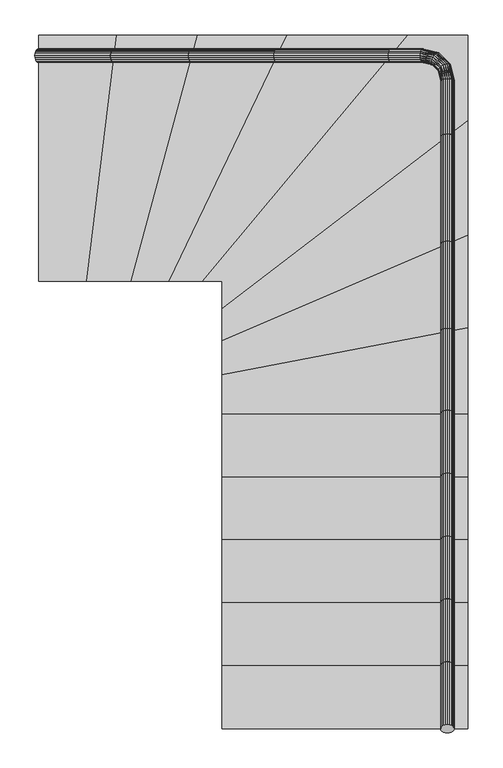
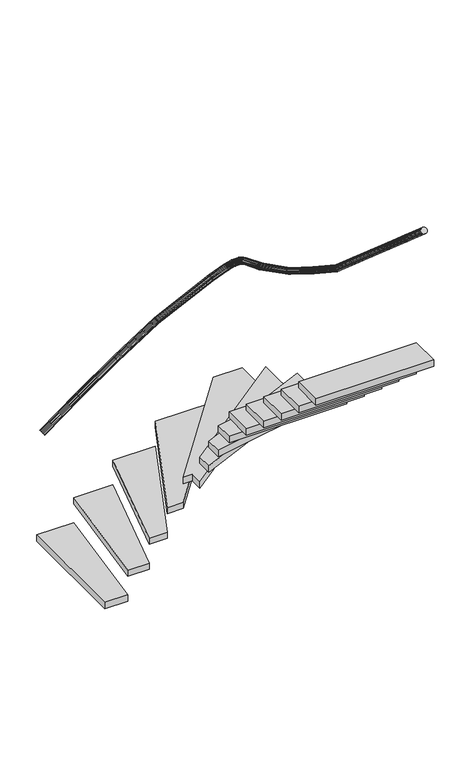
"""IFC4 building model written with IfcOpenShell, lengths in millimetres: stair geometry, 0_3d."""

from ifc_helpers import new_model, si_unit, frame, origin, origin_with_axes, place, context, project, spatial, polyline, outline, extrude, faceted_brep, source, transform, mapped, element, save


def stair_a823ff1d(model_context):
    return source(origin(), model_context, "Body", "SolidModel", [
        extrude(outline(polyline([(1583.4262386, 245.003504), (1583.4262386, 15.003504), (683.4262386, 15.003504), (683.4262386, 245.003504), (1583.4262386, 245.003504)])), frame((0.0, 0.0, 2400.0), z_axis=(0.0, 0.0, 1.0), x_axis=(1.0, 0.0, 0.0)), (0.0, 0.0, 1.0), 50.0),
        faceted_brep([(1303.9880682, 2450.8289277, 1714.5249729), (1301.1493151, 2449.6053406, 1721.0), (1298.310562, 2450.8289277, 1727.4750271), (1295.7496858, 2454.3799157, 1733.3162334), (1293.7173629, 2459.9107093, 1737.951841), (1292.4125313, 2466.8799157, 1740.9280843), (1291.962917, 2474.6053406, 1741.9536279), (1292.4125313, 2482.3307654, 1740.9280843), (1293.7173629, 2489.2999719, 1737.951841), (1295.7496858, 2494.8307654, 1733.3162334), (1298.310562, 2498.3817535, 1727.4750271), (1301.1493151, 2499.6053406, 1721.0), (1303.9880682, 2498.3817535, 1714.5249729), (1306.5489444, 2494.8307654, 1708.6837666), (1308.5812673, 2489.2999719, 1704.048159), (1309.8860989, 2482.3307654, 1701.0719157), (1310.3357132, 2474.6053406, 1700.0463721), (1309.8860989, 2466.8799157, 1701.0719157), (1308.5812673, 2459.9107093, 1704.048159), (1306.5489444, 2454.3799157, 1708.6837666), (1484.6498257, 2181.5291389, 1927.4452788), (1483.4262386, 2178.6155291, 1921.0), (1484.6498257, 2175.7019192, 1914.5547212), (1488.2008138, 2173.0735138, 1908.7403512), (1493.7316073, 2170.9875995, 1904.1260411), (1500.7008138, 2169.64836, 1901.1634716), (1508.4262386, 2169.1868896, 1900.1426397), (1516.1516635, 2169.64836, 1901.1634716), (1523.12087, 2170.9875995, 1904.1260411), (1528.6516635, 2173.0735138, 1908.7403512), (1532.2026516, 2175.7019192, 1914.5547212), (1533.4262386, 2178.6155291, 1921.0), (1532.2026516, 2181.5291389, 1927.4452788), (1528.6516635, 2184.1575443, 1933.2596488), (1523.12087, 2186.2434586, 1937.8739589), (1516.1516635, 2187.5826981, 1940.8365284), (1508.4262386, 2188.0441685, 1941.8573603), (1500.7008138, 2187.5826981, 1940.8365284), (1493.7316073, 2186.2434586, 1937.8739589), (1488.2008138, 2184.1575443, 1933.2596488), (1415.4956, 2449.6053406, 1766.4416225), (1412.8861822, 2450.8289277, 1773.0077883), (1410.5321925, 2454.3799157, 1778.931212), (1408.6640556, 2459.9107093, 1783.6320677), (1407.4646379, 2466.8799157, 1786.6502029), (1407.0513467, 2474.6053406, 1787.6901813), (1407.4646379, 2482.3307654, 1786.6502029), (1408.6640556, 2489.2999719, 1783.6320677), (1410.5321925, 2494.8307654, 1778.931212), (1412.8861822, 2498.3817535, 1773.0077883), (1415.4956, 2499.6053406, 1766.4416225), (1418.1050178, 2498.3817535, 1759.8754567), (1420.4590076, 2494.8307654, 1753.9520329), (1422.3271444, 2489.2999719, 1749.2511773), (1423.5265621, 2482.3307654, 1746.2330421), (1423.9398533, 2474.6053406, 1745.1930636), (1423.5265621, 2466.8799157, 1746.2330421), (1422.3271444, 2459.9107093, 1749.2511773), (1420.4590076, 2454.3799157, 1753.9520329), (1418.1050178, 2450.8289277, 1759.8754567), (1452.4856617, 2441.0391267, 1790.5400059), (1450.1312781, 2443.723795, 1796.7585422), (1449.1829512, 2448.2919784, 1802.3683648), (1449.7335097, 2454.296511, 1806.8203453), (1451.7290611, 2461.1496275, 1809.6786927), (1454.9742669, 2468.1804971, 1810.663612), (1459.1514639, 2474.7008892, 1809.6786927), (1463.8517589, 2480.0725424, 1806.8203453), (1468.6150541, 2483.769642, 1802.3683648), (1472.9750852, 2485.43029, 1796.7585422), (1476.5050619, 2484.8919306, 1790.5400059), (1478.8594454, 2482.2072623, 1784.3214696), (1479.8077724, 2477.639079, 1778.711647), (1479.2572139, 2471.6345463, 1774.2596665), (1477.2616625, 2464.7814298, 1771.4013191), (1474.0164566, 2457.7505602, 1770.4163997), (1469.8392597, 2451.2301681, 1771.4013191), (1465.1389647, 2445.8585149, 1774.2596665), (1460.3756694, 2442.1614153, 1778.711647), (1456.0156384, 2440.5007673, 1784.3214696), (1474.8600248, 2418.6647636, 1816.2051752), (1474.3216654, 2422.1947403, 1822.4237115), (1475.9823134, 2426.5547714, 1828.0335341), (1479.6794129, 2431.3180666, 1832.4855146), (1485.0510662, 2436.0183616, 1835.343862), (1491.5714583, 2440.1955585, 1836.3287814), (1498.6023279, 2443.4407644, 1835.343862), (1505.4554444, 2445.4363158, 1832.4855146), (1511.459977, 2445.9868743, 1828.0335341), (1516.0281603, 2445.0385474, 1822.4237115), (1518.7128287, 2442.6841638, 1816.2051752), (1519.2511881, 2439.1541871, 1809.9866389), (1517.5905401, 2434.7941561, 1804.3768163), (1513.8934405, 2430.0308608, 1799.9248359), (1508.5217873, 2425.3305658, 1797.0664885), (1502.0013951, 2421.1533689, 1796.0815691), (1494.9705256, 2417.908163, 1797.0664885), (1488.1174091, 2415.9126116, 1799.9248359), (1482.1128764, 2415.3620531, 1804.3768163), (1477.5446931, 2416.3103801, 1809.9866389), (1483.4262386, 2381.6747019, 1840.3035586), (1484.6498257, 2384.2841197, 1846.8697244), (1488.2008138, 2386.6381095, 1852.7931482), (1493.7316073, 2388.5062463, 1857.4940039), (1500.7008138, 2389.705664, 1860.512139), (1508.4262386, 2390.1189552, 1861.5521175), (1516.1516635, 2389.705664, 1860.512139), (1523.12087, 2388.5062463, 1857.4940039), (1528.6516635, 2386.6381095, 1852.7931482), (1532.2026516, 2384.2841197, 1846.8697244), (1533.4262386, 2381.6747019, 1840.3035586), (1532.2026516, 2379.0652842, 1833.7373928), (1528.6516635, 2376.7112944, 1827.8139691), (1523.12087, 2374.8431575, 1823.1131134), (1516.1516635, 2373.6437398, 1820.0949783), (1508.4262386, 2373.2304487, 1819.0549998), (1500.7008138, 2373.6437398, 1820.0949783), (1493.7316073, 2374.8431575, 1823.1131134), (1488.2008138, 2376.7112944, 1827.8139691), (1484.6498257, 2379.0652842, 1833.7373928)], [[[0, 1, 2, 3, 4, 5, 6, 7, 8, 9, 10, 11, 12, 13, 14, 15, 16, 17, 18, 19]], [[20, 21, 22, 23, 24, 25, 26, 27, 28, 29, 30, 31, 32, 33, 34, 35, 36, 37, 38, 39]], [[2, 1, 40, 41]], [[3, 2, 41, 42]], [[4, 3, 42, 43]], [[5, 4, 43, 44]], [[6, 5, 44, 45]], [[7, 6, 45, 46]], [[8, 7, 46, 47]], [[9, 8, 47, 48]], [[10, 9, 48, 49]], [[11, 10, 49, 50]], [[12, 11, 50, 51]], [[13, 12, 51, 52]], [[14, 13, 52, 53]], [[15, 14, 53, 54]], [[16, 15, 54, 55]], [[17, 16, 55, 56]], [[18, 17, 56, 57]], [[19, 18, 57, 58]], [[0, 19, 58, 59]], [[1, 0, 59, 40]], [[41, 40, 60]], [[61, 41, 60]], [[42, 41, 61]], [[62, 42, 61]], [[43, 42, 62]], [[63, 43, 62]], [[44, 43, 63]], [[64, 44, 63]], [[45, 44, 64]], [[65, 45, 64]], [[46, 45, 65]], [[66, 46, 65]], [[47, 46, 66]], [[67, 47, 66]], [[48, 47, 67]], [[68, 48, 67]], [[49, 48, 68]], [[69, 49, 68]], [[50, 49, 69]], [[70, 50, 69]], [[51, 50, 70]], [[71, 51, 70]], [[52, 51, 71]], [[72, 52, 71]], [[53, 52, 72]], [[73, 53, 72]], [[54, 53, 73]], [[74, 54, 73]], [[55, 54, 74]], [[75, 55, 74]], [[56, 55, 75]], [[76, 56, 75]], [[57, 56, 76]], [[77, 57, 76]], [[58, 57, 77]], [[78, 58, 77]], [[59, 58, 78]], [[79, 59, 78]], [[40, 59, 79]], [[60, 40, 79]], [[61, 60, 80]], [[81, 61, 80]], [[62, 61, 81]], [[82, 62, 81]], [[63, 62, 82]], [[83, 63, 82]], [[64, 63, 83]], [[84, 64, 83]], [[65, 64, 84]], [[85, 65, 84]], [[66, 65, 85]], [[86, 66, 85]], [[67, 66, 86]], [[87, 67, 86]], [[68, 67, 87]], [[88, 68, 87]], [[69, 68, 88]], [[89, 69, 88]], [[70, 69, 89]], [[90, 70, 89]], [[71, 70, 90]], [[91, 71, 90]], [[72, 71, 91]], [[92, 72, 91]], [[73, 72, 92]], [[93, 73, 92]], [[74, 73, 93]], [[94, 74, 93]], [[75, 74, 94]], [[95, 75, 94]], [[76, 75, 95]], [[96, 76, 95]], [[77, 76, 96]], [[97, 77, 96]], [[78, 77, 97]], [[98, 78, 97]], [[79, 78, 98]], [[99, 79, 98]], [[60, 79, 99]], [[80, 60, 99]], [[81, 80, 100]], [[101, 81, 100]], [[82, 81, 101]], [[102, 82, 101]], [[83, 82, 102]], [[103, 83, 102]], [[84, 83, 103]], [[104, 84, 103]], [[85, 84, 104]], [[105, 85, 104]], [[86, 85, 105]], [[106, 86, 105]], [[87, 86, 106]], [[107, 87, 106]], [[88, 87, 107]], [[108, 88, 107]], [[89, 88, 108]], [[109, 89, 108]], [[90, 89, 109]], [[110, 90, 109]], [[91, 90, 110]], [[111, 91, 110]], [[92, 91, 111]], [[112, 92, 111]], [[93, 92, 112]], [[113, 93, 112]], [[94, 93, 113]], [[114, 94, 113]], [[95, 94, 114]], [[115, 95, 114]], [[96, 95, 115]], [[116, 96, 115]], [[97, 96, 116]], [[117, 97, 116]], [[98, 97, 117]], [[118, 98, 117]], [[99, 98, 118]], [[119, 99, 118]], [[80, 99, 119]], [[100, 80, 119]], [[101, 100, 21, 20]], [[102, 101, 20, 39]], [[103, 102, 39, 38]], [[104, 103, 38, 37]], [[105, 104, 37, 36]], [[106, 105, 36, 35]], [[107, 106, 35, 34]], [[108, 107, 34, 33]], [[109, 108, 33, 32]], [[110, 109, 32, 31]], [[111, 110, 31, 30]], [[112, 111, 30, 29]], [[113, 112, 29, 28]], [[114, 113, 28, 27]], [[115, 114, 27, 26]], [[116, 115, 26, 25]], [[117, 116, 25, 24]], [[118, 117, 24, 23]], [[119, 118, 23, 22]], [[100, 119, 22, 21]]]),
        extrude(outline(polyline([(1583.4262386, 1481.1612025), (1583.4262386, 1165.003504), (683.4262386, 1165.003504), (683.4262386, 1308.8458054), (1583.4262386, 1481.1612025)])), frame((0.0, 0.0, 1400.0), z_axis=(0.0, 0.0, 1.0), x_axis=(1.0, 0.0, 0.0)), (0.0, 0.0, 1.0), 50.0),
        extrude(outline(polyline([(1583.4262386, 935.003504), (1583.4262386, 705.003504), (683.4262386, 705.003504), (683.4262386, 935.003504), (1583.4262386, 935.003504)])), frame((0.0, 0.0, 1800.0), z_axis=(0.0, 0.0, 1.0), x_axis=(1.0, 0.0, 0.0)), (0.0, 0.0, 1.0), 50.0),
        extrude(outline(polyline([(594.7553327, 2549.6053406), (921.0026044, 2549.6053406), (490.0776227, 1649.6053406), (352.0971446, 1649.6053406), (594.7553327, 2549.6053406)])), frame((0.0, 0.0, 400.0), z_axis=(0.0, 0.0, 1.0), x_axis=(1.0, 0.0, 0.0)), (0.0, 0.0, 1.0), 50.0),
        faceted_brep([(888.5488665, 2450.8289277, 1514.822011), (885.0921893, 2449.6053406, 1521.0), (881.635512, 2450.8289277, 1527.177989), (878.5171983, 2454.3799157, 1532.7512333), (876.0424906, 2459.9107093, 1537.1741851), (874.4536305, 2466.8799157, 1540.013895), (873.9061466, 2474.6053406, 1540.9923923), (874.4536305, 2482.3307654, 1540.013895), (876.0424906, 2489.2999719, 1537.1741851), (878.5171983, 2494.8307654, 1532.7512333), (881.635512, 2498.3817535, 1527.177989), (885.0921893, 2499.6053406, 1521.0), (888.5488665, 2498.3817535, 1514.822011), (891.6671802, 2494.8307654, 1509.2487667), (894.1418879, 2489.2999719, 1504.8258149), (895.730748, 2482.3307654, 1501.986105), (896.2782319, 2474.6053406, 1501.0076077), (895.730748, 2466.8799157, 1501.986105), (894.1418879, 2459.9107093, 1504.8258149), (891.6671802, 2454.3799157, 1509.2487667), (1298.310562, 2450.8289277, 1727.4750271), (1301.1493151, 2449.6053406, 1721.0), (1303.9880682, 2450.8289277, 1714.5249729), (1306.5489444, 2454.3799157, 1708.6837666), (1308.5812673, 2459.9107093, 1704.048159), (1309.8860989, 2466.8799157, 1701.0719157), (1310.3357132, 2474.6053406, 1700.0463721), (1309.8860989, 2482.3307654, 1701.0719157), (1308.5812673, 2489.2999719, 1704.048159), (1306.5489444, 2494.8307654, 1708.6837666), (1303.9880682, 2498.3817535, 1714.5249729), (1301.1493151, 2499.6053406, 1721.0), (1298.310562, 2498.3817535, 1727.4750271), (1295.7496858, 2494.8307654, 1733.3162334), (1293.7173629, 2489.2999719, 1737.951841), (1292.4125313, 2482.3307654, 1740.9280843), (1291.962917, 2474.6053406, 1741.9536279), (1292.4125313, 2466.8799157, 1740.9280843), (1293.7173629, 2459.9107093, 1737.951841), (1295.7496858, 2454.3799157, 1733.3162334)], [[[0, 1, 2, 3, 4, 5, 6, 7, 8, 9, 10, 11, 12, 13, 14, 15, 16, 17, 18, 19]], [[20, 21, 22, 23, 24, 25, 26, 27, 28, 29, 30, 31, 32, 33, 34, 35, 36, 37, 38, 39]], [[2, 1, 21, 20]], [[3, 2, 20, 39]], [[4, 3, 39, 38]], [[5, 4, 38, 37]], [[6, 5, 37, 36]], [[7, 6, 36, 35]], [[8, 7, 35, 34]], [[9, 8, 34, 33]], [[10, 9, 33, 32]], [[11, 10, 32, 31]], [[12, 11, 31, 30]], [[13, 12, 30, 29]], [[14, 13, 29, 28]], [[15, 14, 28, 27]], [[16, 15, 27, 26]], [[17, 16, 26, 25]], [[18, 17, 25, 24]], [[19, 18, 24, 23]], [[0, 19, 23, 22]], [[1, 0, 22, 21]]]),
        extrude(outline(polyline([(1.2235871, -7.0656631), (0.0, 0.0), (1.2235871, 7.0656631), (4.7745752, 13.4396897), (10.3053687, 18.4981459), (17.2745752, 21.7458748), (25.0, 22.8649659), (32.7254249, 21.7458748), (39.6946314, 18.4981459), (45.2254249, 13.4396897), (48.776413, 7.0656631), (50.0, 0.0), (48.776413, -7.0656631), (45.2254249, -13.4396898), (39.6946314, -18.498146), (32.7254249, -21.7458748), (25.0, -22.864966), (17.2745752, -21.7458748), (10.3053687, -18.498146), (4.7745752, -13.4396898), (1.2235871, -7.0656631)])), frame((1483.4262386, 245.003504, 3321.0), z_axis=(0.0, -0.7546055221635334, 0.6561787149247537), x_axis=(1.0, 0.0, 0.0)), (0.0, 0.0, 1.0), 304.7950131),
        faceted_brep([(1484.6498257, 1160.7155489, 2515.3652703), (1483.4262386, 1165.003504, 2521.0), (1484.6498257, 1169.2914591, 2526.6347297), (1488.2008138, 1173.1596792, 2531.7178929), (1493.7316073, 1176.2295162, 2535.751914), (1500.7008138, 1178.2004728, 2538.341915), (1508.4262386, 1178.8796182, 2539.2343685), (1516.1516635, 1178.2004728, 2538.341915), (1523.12087, 1176.2295162, 2535.751914), (1528.6516635, 1173.1596792, 2531.7178929), (1532.2026516, 1169.2914591, 2526.6347297), (1533.4262386, 1165.003504, 2521.0), (1532.2026516, 1160.7155489, 2515.3652703), (1528.6516635, 1156.8473287, 2510.2821071), (1523.12087, 1153.7774918, 2506.248086), (1516.1516635, 1151.8065351, 2503.658085), (1508.4262386, 1151.1273898, 2502.7656315), (1500.7008138, 1151.8065351, 2503.658085), (1493.7316073, 1153.7774918, 2506.248086), (1488.2008138, 1156.8473287, 2510.2821071), (1484.6498257, 939.6398417, 2726.3317884), (1483.4262386, 935.003504, 2721.0), (1484.6498257, 930.3671663, 2715.6682116), (1488.2008138, 926.1846656, 2710.8583359), (1493.7316073, 922.8654143, 2707.0411969), (1500.7008138, 920.7343238, 2704.5904428), (1508.4262386, 920.0, 2703.7459704), (1516.1516635, 920.7343238, 2704.5904428), (1523.12087, 922.8654143, 2707.0411969), (1528.6516635, 926.1846656, 2710.8583359), (1532.2026516, 930.3671663, 2715.6682116), (1533.4262386, 935.003504, 2721.0), (1532.2026516, 939.6398417, 2726.3317884), (1528.6516635, 943.8223423, 2731.1416641), (1523.12087, 947.1415936, 2734.9588031), (1516.1516635, 949.2726842, 2737.4095572), (1508.4262386, 950.0070079, 2738.2540296), (1500.7008138, 949.2726842, 2737.4095572), (1493.7316073, 947.1415936, 2734.9588031), (1488.2008138, 943.8223423, 2731.1416641)], [[[0, 1, 2, 3, 4, 5, 6, 7, 8, 9, 10, 11, 12, 13, 14, 15, 16, 17, 18, 19]], [[20, 21, 22, 23, 24, 25, 26, 27, 28, 29, 30, 31, 32, 33, 34, 35, 36, 37, 38, 39]], [[2, 1, 21, 20]], [[3, 2, 20, 39]], [[4, 3, 39, 38]], [[5, 4, 38, 37]], [[6, 5, 37, 36]], [[7, 6, 36, 35]], [[8, 7, 35, 34]], [[9, 8, 34, 33]], [[10, 9, 33, 32]], [[11, 10, 32, 31]], [[12, 11, 31, 30]], [[13, 12, 30, 29]], [[14, 13, 29, 28]], [[15, 14, 28, 27]], [[16, 15, 27, 26]], [[17, 16, 26, 25]], [[18, 17, 25, 24]], [[19, 18, 24, 23]], [[0, 19, 23, 22]], [[1, 0, 22, 21]]]),
        extrude(outline(polyline([(1.2235871, -7.0656631), (0.0, 0.0), (1.2235871, 7.0656631), (4.7745752, 13.4396897), (10.3053687, 18.4981459), (17.2745752, 21.7458748), (25.0, 22.8649659), (32.7254249, 21.7458748), (39.6946314, 18.4981459), (45.2254249, 13.4396897), (48.776413, 7.0656631), (50.0, 0.0), (48.776413, -7.0656631), (45.2254249, -13.4396898), (39.6946314, -18.498146), (32.7254249, -21.7458748), (25.0, -22.864966), (17.2745752, -21.7458748), (10.3053687, -18.498146), (4.7745752, -13.4396898), (1.2235871, -7.0656631)])), frame((1483.4262386, 475.003504, 3121.0), z_axis=(0.0, -0.7546055221635319, 0.6561787149247553), x_axis=(1.0, 0.0, 0.0)), (0.0, 0.0, 1.0), 304.7950131),
        faceted_brep([(1484.6498257, 1782.2333607, 2114.8463761), (1483.4262386, 1785.7199202, 2121.0), (1484.6498257, 1789.2064798, 2127.1536239), (1488.2008138, 1792.3517506, 2132.7048881), (1493.7316073, 1794.8478516, 2137.1103964), (1500.7008138, 1796.4504471, 2139.9389068), (1508.4262386, 1797.0026639, 2140.9135451), (1516.1516635, 1796.4504471, 2139.9389068), (1523.12087, 1794.8478516, 2137.1103964), (1528.6516635, 1792.3517506, 2132.7048881), (1532.2026516, 1789.2064798, 2127.1536239), (1533.4262386, 1785.7199202, 2121.0), (1532.2026516, 1782.2333607, 2114.8463761), (1528.6516635, 1779.0880899, 2109.2951119), (1523.12087, 1776.5919889, 2104.8896036), (1516.1516635, 1774.9893933, 2102.0610932), (1508.4262386, 1774.4371766, 2101.0864549), (1500.7008138, 1774.9893933, 2102.0610932), (1493.7316073, 1776.5919889, 2104.8896036), (1488.2008138, 1779.0880899, 2109.2951119), (1484.6498257, 1470.6307046, 2326.9387983), (1483.4262386, 1466.8015861, 2321.0), (1484.6498257, 1462.9724676, 2315.0612017), (1488.2008138, 1459.5181699, 2309.7037343), (1493.7316073, 1456.7768237, 2305.4520241), (1500.7008138, 1455.0167712, 2302.7222581), (1508.4262386, 1454.4102984, 2301.7816448), (1516.1516635, 1455.0167712, 2302.7222581), (1523.12087, 1456.7768237, 2305.4520241), (1528.6516635, 1459.5181699, 2309.7037343), (1532.2026516, 1462.9724676, 2315.0612017), (1533.4262386, 1466.8015861, 2321.0), (1532.2026516, 1470.6307046, 2326.9387983), (1528.6516635, 1474.0850023, 2332.2962657), (1523.12087, 1476.8263485, 2336.5479759), (1516.1516635, 1478.5864011, 2339.2777419), (1508.4262386, 1479.1928739, 2340.2183552), (1500.7008138, 1478.5864011, 2339.2777419), (1493.7316073, 1476.8263485, 2336.5479759), (1488.2008138, 1474.0850023, 2332.2962657)], [[[0, 1, 2, 3, 4, 5, 6, 7, 8, 9, 10, 11, 12, 13, 14, 15, 16, 17, 18, 19]], [[20, 21, 22, 23, 24, 25, 26, 27, 28, 29, 30, 31, 32, 33, 34, 35, 36, 37, 38, 39]], [[2, 1, 21, 20]], [[3, 2, 20, 39]], [[4, 3, 39, 38]], [[5, 4, 38, 37]], [[6, 5, 37, 36]], [[7, 6, 36, 35]], [[8, 7, 35, 34]], [[9, 8, 34, 33]], [[10, 9, 33, 32]], [[11, 10, 32, 31]], [[12, 11, 31, 30]], [[13, 12, 30, 29]], [[14, 13, 29, 28]], [[15, 14, 28, 27]], [[16, 15, 27, 26]], [[17, 16, 26, 25]], [[18, 17, 25, 24]], [[19, 18, 24, 23]], [[0, 19, 23, 22]], [[1, 0, 22, 21]]]),
        extrude(outline(polyline([(1583.4262386, 475.003504), (1583.4262386, 245.003504), (683.4262386, 245.003504), (683.4262386, 475.003504), (1583.4262386, 475.003504)])), frame((0.0, 0.0, 2200.0), z_axis=(0.0, 0.0, 1.0), x_axis=(1.0, 0.0, 0.0)), (0.0, 0.0, 1.0), 50.0),
        extrude(outline(polyline([(1583.4262386, 1817.8101985), (1583.4262386, 1481.1612025), (683.4262386, 1308.8458054), (683.4262386, 1432.7268587), (1583.4262386, 1817.8101985)])), frame((0.0, 0.0, 1200.0), z_axis=(0.0, 0.0, 1.0), x_axis=(1.0, 0.0, 0.0)), (0.0, 0.0, 1.0), 50.0),
        extrude(outline(polyline([(298.2634034, 2549.6053406), (594.7553327, 2549.6053406), (352.0971446, 1649.6053406), (188.5890739, 1649.6053406), (298.2634034, 2549.6053406)])), frame((0.0, 0.0, 200.0), z_axis=(0.0, 0.0, 1.0), x_axis=(1.0, 0.0, 0.0)), (0.0, 0.0, 1.0), 50.0),
        extrude(outline(polyline([(921.0026044, 2549.6053406), (1363.6695948, 2549.6053406), (613.4262386, 1649.6053406), (490.0776227, 1649.6053406), (921.0026044, 2549.6053406)])), frame((0.0, 0.0, 600.0), z_axis=(0.0, 0.0, 1.0), x_axis=(1.0, 0.0, 0.0)), (0.0, 0.0, 1.0), 50.0),
        extrude(outline(polyline([(1.2235871, -7.0656631), (0.0, 0.0), (1.2235871, 7.0656631), (4.7745752, 13.4396897), (10.3053687, 18.4981459), (17.2745752, 21.7458748), (25.0, 22.8649659), (32.7254249, 21.7458748), (39.6946314, 18.4981459), (45.2254249, 13.4396897), (48.776413, 7.0656631), (50.0, 0.0), (48.776413, -7.0656631), (45.2254249, -13.4396898), (39.6946314, -18.498146), (32.7254249, -21.7458748), (25.0, -22.864966), (17.2745752, -21.7458748), (10.3053687, -18.498146), (4.7745752, -13.4396898), (1.2235871, -7.0656631)])), frame((1483.4262386, 935.003504, 2721.0), z_axis=(0.0, -0.7546055221635329, 0.6561787149247542), x_axis=(1.0, 0.0, 0.0)), (0.0, 0.0, 1.0), 304.7950131),
        extrude(outline(polyline([(1583.4262386, 705.003504), (1583.4262386, 475.003504), (683.4262386, 475.003504), (683.4262386, 705.003504), (1583.4262386, 705.003504)])), frame((0.0, 0.0, 2000.0), z_axis=(0.0, 0.0, 1.0), x_axis=(1.0, 0.0, 0.0)), (0.0, 0.0, 1.0), 50.0),
        extrude(outline(polyline([(1583.4262386, 1165.003504), (1583.4262386, 935.003504), (683.4262386, 935.003504), (683.4262386, 1165.003504), (1583.4262386, 1165.003504)])), frame((0.0, 0.0, 1600.0), z_axis=(0.0, 0.0, 1.0), x_axis=(1.0, 0.0, 0.0)), (0.0, 0.0, 1.0), 50.0),
        extrude(outline(polyline([(13.4262386, 2549.6053406), (298.2634034, 2549.6053406), (188.5890739, 1649.6053406), (13.4262386, 1649.6053406), (13.4262386, 2549.6053406)])), origin_with_axes(), (0.0, 0.0, 1.0), 50.0),
        faceted_brep([(1484.6498257, 2175.7019192, 1914.5547212), (1483.4262386, 2178.6155291, 1921.0), (1484.6498257, 2181.5291389, 1927.4452788), (1488.2008138, 2184.1575443, 1933.2596488), (1493.7316073, 2186.2434586, 1937.8739589), (1500.7008138, 2187.5826981, 1940.8365284), (1508.4262386, 2188.0441685, 1941.8573603), (1516.1516635, 2187.5826981, 1940.8365284), (1523.12087, 2186.2434586, 1937.8739589), (1528.6516635, 2184.1575443, 1933.2596488), (1532.2026516, 2181.5291389, 1927.4452788), (1533.4262386, 2178.6155291, 1921.0), (1532.2026516, 2175.7019192, 1914.5547212), (1528.6516635, 2173.0735138, 1908.7403512), (1523.12087, 2170.9875995, 1904.1260411), (1516.1516635, 2169.64836, 1901.1634716), (1508.4262386, 2169.1868896, 1900.1426397), (1500.7008138, 2169.64836, 1901.1634716), (1493.7316073, 2170.9875995, 1904.1260411), (1488.2008138, 2173.0735138, 1908.7403512), (1484.6498257, 1789.2064798, 2127.1536239), (1483.4262386, 1785.7199202, 2121.0), (1484.6498257, 1782.2333607, 2114.8463761), (1488.2008138, 1779.0880899, 2109.2951119), (1493.7316073, 1776.5919889, 2104.8896036), (1500.7008138, 1774.9893933, 2102.0610932), (1508.4262386, 1774.4371766, 2101.0864549), (1516.1516635, 1774.9893933, 2102.0610932), (1523.12087, 1776.5919889, 2104.8896036), (1528.6516635, 1779.0880899, 2109.2951119), (1532.2026516, 1782.2333607, 2114.8463761), (1533.4262386, 1785.7199202, 2121.0), (1532.2026516, 1789.2064798, 2127.1536239), (1528.6516635, 1792.3517506, 2132.7048881), (1523.12087, 1794.8478516, 2137.1103964), (1516.1516635, 1796.4504471, 2139.9389068), (1508.4262386, 1797.0026639, 2140.9135451), (1500.7008138, 1796.4504471, 2139.9389068), (1493.7316073, 1794.8478516, 2137.1103964), (1488.2008138, 1792.3517506, 2132.7048881)], [[[0, 1, 2, 3, 4, 5, 6, 7, 8, 9, 10, 11, 12, 13, 14, 15, 16, 17, 18, 19]], [[20, 21, 22, 23, 24, 25, 26, 27, 28, 29, 30, 31, 32, 33, 34, 35, 36, 37, 38, 39]], [[2, 1, 21, 20]], [[3, 2, 20, 39]], [[4, 3, 39, 38]], [[5, 4, 38, 37]], [[6, 5, 37, 36]], [[7, 6, 36, 35]], [[8, 7, 35, 34]], [[9, 8, 34, 33]], [[10, 9, 33, 32]], [[11, 10, 32, 31]], [[12, 11, 31, 30]], [[13, 12, 30, 29]], [[14, 13, 29, 28]], [[15, 14, 28, 27]], [[16, 15, 27, 26]], [[17, 16, 26, 25]], [[18, 17, 25, 24]], [[19, 18, 24, 23]], [[0, 19, 23, 22]], [[1, 0, 22, 21]]]),
        faceted_brep([(1484.6498257, 1462.9724676, 2315.0612017), (1483.4262386, 1466.8015861, 2321.0), (1484.6498257, 1470.6307046, 2326.9387983), (1488.2008138, 1474.0850023, 2332.2962657), (1493.7316073, 1476.8263485, 2336.5479759), (1500.7008138, 1478.5864011, 2339.2777419), (1508.4262386, 1479.1928739, 2340.2183552), (1516.1516635, 1478.5864011, 2339.2777419), (1523.12087, 1476.8263485, 2336.5479759), (1528.6516635, 1474.0850023, 2332.2962657), (1532.2026516, 1470.6307046, 2326.9387983), (1533.4262386, 1466.8015861, 2321.0), (1532.2026516, 1462.9724676, 2315.0612017), (1528.6516635, 1459.5181699, 2309.7037343), (1523.12087, 1456.7768237, 2305.4520241), (1516.1516635, 1455.0167712, 2302.7222581), (1508.4262386, 1454.4102984, 2301.7816448), (1500.7008138, 1455.0167712, 2302.7222581), (1493.7316073, 1456.7768237, 2305.4520241), (1488.2008138, 1459.5181699, 2309.7037343), (1484.6498257, 1169.2914591, 2526.6347297), (1483.4262386, 1165.003504, 2521.0), (1484.6498257, 1160.7155489, 2515.3652703), (1488.2008138, 1156.8473287, 2510.2821071), (1493.7316073, 1153.7774918, 2506.248086), (1500.7008138, 1151.8065351, 2503.658085), (1508.4262386, 1151.1273898, 2502.7656315), (1516.1516635, 1151.8065351, 2503.658085), (1523.12087, 1153.7774918, 2506.248086), (1528.6516635, 1156.8473287, 2510.2821071), (1532.2026516, 1160.7155489, 2515.3652703), (1533.4262386, 1165.003504, 2521.0), (1532.2026516, 1169.2914591, 2526.6347297), (1528.6516635, 1173.1596792, 2531.7178929), (1523.12087, 1176.2295162, 2535.751914), (1516.1516635, 1178.2004728, 2538.341915), (1508.4262386, 1178.8796182, 2539.2343685), (1500.7008138, 1178.2004728, 2538.341915), (1493.7316073, 1176.2295162, 2535.751914), (1488.2008138, 1173.1596792, 2531.7178929)], [[[0, 1, 2, 3, 4, 5, 6, 7, 8, 9, 10, 11, 12, 13, 14, 15, 16, 17, 18, 19]], [[20, 21, 22, 23, 24, 25, 26, 27, 28, 29, 30, 31, 32, 33, 34, 35, 36, 37, 38, 39]], [[2, 1, 21, 20]], [[3, 2, 20, 39]], [[4, 3, 39, 38]], [[5, 4, 38, 37]], [[6, 5, 37, 36]], [[7, 6, 36, 35]], [[8, 7, 35, 34]], [[9, 8, 34, 33]], [[10, 9, 33, 32]], [[11, 10, 32, 31]], [[12, 11, 31, 30]], [[13, 12, 30, 29]], [[14, 13, 29, 28]], [[15, 14, 28, 27]], [[16, 15, 27, 26]], [[17, 16, 26, 25]], [[18, 17, 25, 24]], [[19, 18, 24, 23]], [[0, 19, 23, 22]], [[1, 0, 22, 21]]]),
        faceted_brep([(578.4755263, 2450.8289277, 1315.1343723), (574.5338171, 2449.6053406, 1321.0), (570.5921078, 2450.8289277, 1326.8656277), (567.0362404, 2454.3799157, 1332.1570869), (564.2142882, 2459.9107093, 1336.3564127), (562.4024833, 2466.8799157, 1339.0525459), (561.7781779, 2474.6053406, 1339.98157), (562.4024833, 2482.3307654, 1339.0525459), (564.2142882, 2489.2999719, 1336.3564127), (567.0362404, 2494.8307654, 1332.1570869), (570.5921078, 2498.3817535, 1326.8656277), (574.5338171, 2499.6053406, 1321.0), (578.4755263, 2498.3817535, 1315.1343723), (582.0313937, 2494.8307654, 1309.8429131), (584.8533459, 2489.2999719, 1305.6435873), (586.6651508, 2482.3307654, 1302.9474541), (587.2894563, 2474.6053406, 1302.01843), (586.6651508, 2466.8799157, 1302.9474541), (584.8533459, 2459.9107093, 1305.6435873), (582.0313937, 2454.3799157, 1309.8429131), (881.635512, 2450.8289277, 1527.177989), (885.0921893, 2449.6053406, 1521.0), (888.5488665, 2450.8289277, 1514.822011), (891.6671802, 2454.3799157, 1509.2487667), (894.1418879, 2459.9107093, 1504.8258149), (895.730748, 2466.8799157, 1501.986105), (896.2782319, 2474.6053406, 1501.0076077), (895.730748, 2482.3307654, 1501.986105), (894.1418879, 2489.2999719, 1504.8258149), (891.6671802, 2494.8307654, 1509.2487667), (888.5488665, 2498.3817535, 1514.822011), (885.0921893, 2499.6053406, 1521.0), (881.635512, 2498.3817535, 1527.177989), (878.5171983, 2494.8307654, 1532.7512333), (876.0424906, 2489.2999719, 1537.1741851), (874.4536305, 2482.3307654, 1540.013895), (873.9061466, 2474.6053406, 1540.9923923), (874.4536305, 2466.8799157, 1540.013895), (876.0424906, 2459.9107093, 1537.1741851), (878.5171983, 2454.3799157, 1532.7512333)], [[[0, 1, 2, 3, 4, 5, 6, 7, 8, 9, 10, 11, 12, 13, 14, 15, 16, 17, 18, 19]], [[20, 21, 22, 23, 24, 25, 26, 27, 28, 29, 30, 31, 32, 33, 34, 35, 36, 37, 38, 39]], [[2, 1, 21, 20]], [[3, 2, 20, 39]], [[4, 3, 39, 38]], [[5, 4, 38, 37]], [[6, 5, 37, 36]], [[7, 6, 36, 35]], [[8, 7, 35, 34]], [[9, 8, 34, 33]], [[10, 9, 33, 32]], [[11, 10, 32, 31]], [[12, 11, 31, 30]], [[13, 12, 30, 29]], [[14, 13, 29, 28]], [[15, 14, 28, 27]], [[16, 15, 27, 26]], [[17, 16, 26, 25]], [[18, 17, 25, 24]], [[19, 18, 24, 23]], [[0, 19, 23, 22]], [[1, 0, 22, 21]]]),
        faceted_brep([(17.5751746, 2450.8289277, 915.2807409), (13.4262386, 2449.6053406, 921.0), (9.2773027, 2450.8289277, 926.7192591), (5.5344936, 2454.3799157, 931.8786773), (2.5641834, 2459.9107093, 935.9732148), (0.6571269, 2466.8799157, 938.6020697), (0.0, 2474.6053406, 939.5079114), (0.6571269, 2482.3307654, 938.6020697), (2.5641834, 2489.2999719, 935.9732148), (5.5344936, 2494.8307654, 931.8786773), (9.2773027, 2498.3817535, 926.7192591), (13.4262386, 2499.6053406, 921.0), (17.5751746, 2498.3817535, 915.2807409), (21.3179837, 2494.8307654, 910.1213227), (24.2882939, 2489.2999719, 906.0267852), (26.1953504, 2482.3307654, 903.3979303), (26.8524773, 2474.6053406, 902.4920886), (26.1953504, 2466.8799157, 903.3979303), (24.2882939, 2459.9107093, 906.0267852), (21.3179837, 2454.3799157, 910.1213227), (285.0217384, 2450.8289277, 1126.7532082), (289.123876, 2449.6053406, 1121.0), (293.2260135, 2450.8289277, 1115.2467918), (296.9266053, 2454.3799157, 1110.0567478), (299.8634116, 2459.9107093, 1105.9379055), (301.7489573, 2466.8799157, 1103.2934459), (302.398672, 2474.6053406, 1102.3822273), (301.7489573, 2482.3307654, 1103.2934459), (299.8634116, 2489.2999719, 1105.9379055), (296.9266053, 2494.8307654, 1110.0567478), (293.2260135, 2498.3817535, 1115.2467918), (289.123876, 2499.6053406, 1121.0), (285.0217384, 2498.3817535, 1126.7532082), (281.3211466, 2494.8307654, 1131.9432522), (278.3843403, 2489.2999719, 1136.0620945), (276.4987947, 2482.3307654, 1138.7065541), (275.8490799, 2474.6053406, 1139.6177727), (276.4987947, 2466.8799157, 1138.7065541), (278.3843403, 2459.9107093, 1136.0620945), (281.3211466, 2454.3799157, 1131.9432522)], [[[0, 1, 2, 3, 4, 5, 6, 7, 8, 9, 10, 11, 12, 13, 14, 15, 16, 17, 18, 19]], [[20, 21, 22, 23, 24, 25, 26, 27, 28, 29, 30, 31, 32, 33, 34, 35, 36, 37, 38, 39]], [[2, 1, 21, 20]], [[3, 2, 20, 39]], [[4, 3, 39, 38]], [[5, 4, 38, 37]], [[6, 5, 37, 36]], [[7, 6, 36, 35]], [[8, 7, 35, 34]], [[9, 8, 34, 33]], [[10, 9, 33, 32]], [[11, 10, 32, 31]], [[12, 11, 31, 30]], [[13, 12, 30, 29]], [[14, 13, 29, 28]], [[15, 14, 28, 27]], [[16, 15, 27, 26]], [[17, 16, 26, 25]], [[18, 17, 25, 24]], [[19, 18, 24, 23]], [[0, 19, 23, 22]], [[1, 0, 22, 21]]]),
        extrude(outline(polyline([(1.2235871, -7.0656631), (0.0, 0.0), (1.2235871, 7.0656631), (4.7745752, 13.4396897), (10.3053687, 18.4981459), (17.2745752, 21.7458748), (25.0, 22.8649659), (32.7254249, 21.7458748), (39.6946314, 18.4981459), (45.2254249, 13.4396897), (48.776413, 7.0656631), (50.0, 0.0), (48.776413, -7.0656631), (45.2254249, -13.4396898), (39.6946314, -18.498146), (32.7254249, -21.7458748), (25.0, -22.864966), (17.2745752, -21.7458748), (10.3053687, -18.498146), (4.7745752, -13.4396898), (1.2235871, -7.0656631)])), frame((1483.4262386, 705.003504, 2921.0), z_axis=(0.0, -0.7546055221635312, 0.6561787149247563), x_axis=(1.0, 0.0, 0.0)), (0.0, 0.0, 1.0), 304.7950131),
        extrude(outline(polyline([(1363.6695948, 2549.6053406), (1583.4262386, 2549.6053406), (1583.4262386, 2235.7982735), (683.4262386, 1549.6053406), (683.4262386, 1649.6053406), (613.4262386, 1649.6053406), (1363.6695948, 2549.6053406)])), frame((0.0, 0.0, 800.0), z_axis=(0.0, 0.0, 1.0), x_axis=(1.0, 0.0, 0.0)), (0.0, 0.0, 1.0), 50.0),
        faceted_brep([(293.2260135, 2450.8289277, 1115.2467918), (289.123876, 2449.6053406, 1121.0), (285.0217384, 2450.8289277, 1126.7532082), (281.3211466, 2454.3799157, 1131.9432522), (278.3843403, 2459.9107093, 1136.0620945), (276.4987947, 2466.8799157, 1138.7065541), (275.8490799, 2474.6053406, 1139.6177727), (276.4987947, 2482.3307654, 1138.7065541), (278.3843403, 2489.2999719, 1136.0620945), (281.3211466, 2494.8307654, 1131.9432522), (285.0217384, 2498.3817535, 1126.7532082), (289.123876, 2499.6053406, 1121.0), (293.2260135, 2498.3817535, 1115.2467918), (296.9266053, 2494.8307654, 1110.0567478), (299.8634116, 2489.2999719, 1105.9379055), (301.7489573, 2482.3307654, 1103.2934459), (302.398672, 2474.6053406, 1102.3822273), (301.7489573, 2466.8799157, 1103.2934459), (299.8634116, 2459.9107093, 1105.9379055), (296.9266053, 2454.3799157, 1110.0567478), (570.5921078, 2450.8289277, 1326.8656277), (574.5338171, 2449.6053406, 1321.0), (578.4755263, 2450.8289277, 1315.1343723), (582.0313937, 2454.3799157, 1309.8429131), (584.8533459, 2459.9107093, 1305.6435873), (586.6651508, 2466.8799157, 1302.9474541), (587.2894563, 2474.6053406, 1302.01843), (586.6651508, 2482.3307654, 1302.9474541), (584.8533459, 2489.2999719, 1305.6435873), (582.0313937, 2494.8307654, 1309.8429131), (578.4755263, 2498.3817535, 1315.1343723), (574.5338171, 2499.6053406, 1321.0), (570.5921078, 2498.3817535, 1326.8656277), (567.0362404, 2494.8307654, 1332.1570869), (564.2142882, 2489.2999719, 1336.3564127), (562.4024833, 2482.3307654, 1339.0525459), (561.7781779, 2474.6053406, 1339.98157), (562.4024833, 2466.8799157, 1339.0525459), (564.2142882, 2459.9107093, 1336.3564127), (567.0362404, 2454.3799157, 1332.1570869)], [[[0, 1, 2, 3, 4, 5, 6, 7, 8, 9, 10, 11, 12, 13, 14, 15, 16, 17, 18, 19]], [[20, 21, 22, 23, 24, 25, 26, 27, 28, 29, 30, 31, 32, 33, 34, 35, 36, 37, 38, 39]], [[2, 1, 21, 20]], [[3, 2, 20, 39]], [[4, 3, 39, 38]], [[5, 4, 38, 37]], [[6, 5, 37, 36]], [[7, 6, 36, 35]], [[8, 7, 35, 34]], [[9, 8, 34, 33]], [[10, 9, 33, 32]], [[11, 10, 32, 31]], [[12, 11, 31, 30]], [[13, 12, 30, 29]], [[14, 13, 29, 28]], [[15, 14, 28, 27]], [[16, 15, 27, 26]], [[17, 16, 26, 25]], [[18, 17, 25, 24]], [[19, 18, 24, 23]], [[0, 19, 23, 22]], [[1, 0, 22, 21]]]),
        extrude(outline(polyline([(1583.4262386, 2235.7982735), (1583.4262386, 1817.8101985), (683.4262386, 1432.7268587), (683.4262386, 1549.6053406), (1583.4262386, 2235.7982735)])), frame((0.0, 0.0, 1000.0), z_axis=(0.0, 0.0, 1.0), x_axis=(1.0, 0.0, 0.0)), (0.0, 0.0, 1.0), 50.0),
    ])


if __name__ == "__main__":
    model = new_model("IFC4")
    model_context = context("Model", 3, world=origin())
    ifc_project = project(units=[si_unit("LENGTHUNIT", "METRE", prefix="MILLI")], contexts=[model_context])
    site = spatial("IfcSite", under=ifc_project)
    building = spatial("IfcBuilding", under=site)
    placement = place(None, origin())
    stair_shape = stair_a823ff1d(model_context)
    element("IfcStair", 1, ObjectType="0_3d", at=placement, inside=building, context=model_context, shape_type="MappedRepresentation", body=[
        mapped(stair_shape, transform((0.0, 0.0, 0.0), x_axis=(1.0, 0.0, 0.0), y_axis=(0.0, 1.0, 0.0), z_axis=(0.0, 0.0, 1.0))),
    ])
    save(model, "model.ifc")

# Revit data of these elements
# Element 1 (IfcStair, "0_3d")
#   Materials on its faces: "*1", "weiss"
# Materials
#   "*1": class "Unassigned", colour RGB 175 175 175, transparency 0
#   "weiss": class "Unassigned", colour RGB 255 255 255, transparency 0
